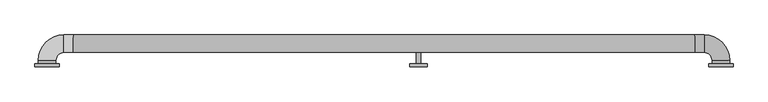
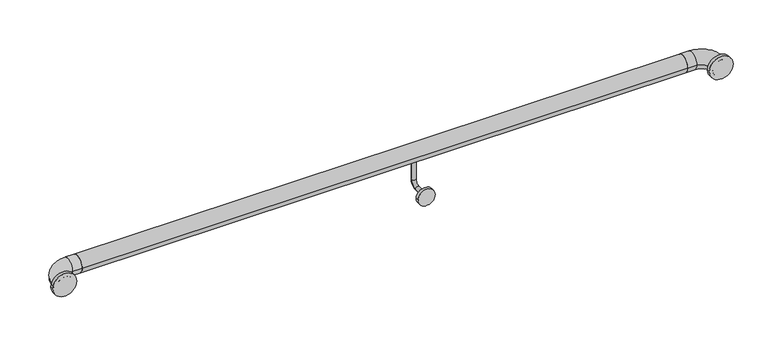
"""IFC4 building model written with IfcOpenShell, lengths in millimetres: railing geometry."""

from ifc_helpers import new_model, si_unit, point, frame, frame_2d, origin, place, context, project, spatial, circle_curve, ellipse_curve, trimmed, segment, composite_curve, outline, extrude, source, transform, mapped, element, save
from ifc_brep_helpers import plane_surface, cylinder_surface, revolved_surface, advanced_brep


def railing_d82230a8(model_context):
    return source(origin(), model_context, "Body", "SolidModel", [
        extrude(outline(composite_curve([segment(trimmed(circle_curve(frame_2d((32728.1400611, 874.6)), 25.4), [point((32753.5400611, 874.6))], [point((32702.7400611, 874.6))], False, "CARTESIAN"), True, "CONTINUOUS"), segment(trimmed(circle_curve(frame_2d((32728.1400611, 874.6)), 25.4), [point((32702.7400611, 874.6))], [point((32753.5400611, 874.6))], False, "CARTESIAN"), True, "CONTINUOUS")], self_intersect=False)), frame((9766.6129185, 0.0, 0.0), z_axis=(1.0, 0.0, 0.0), x_axis=(0.0, 1.0, 0.0)), (0.0, 0.0, 1.0), 1800.0),
        extrude(outline(composite_curve([segment(trimmed(circle_curve(frame_2d((773.2, 10766.6129185)), 25.4), [point((773.2, 10792.0129185))], [point((773.2, 10741.2129185))], False, "CARTESIAN"), True, "CONTINUOUS"), segment(trimmed(circle_curve(frame_2d((773.2, 10766.6129185)), 25.4), [point((773.2, 10741.2129185))], [point((773.2, 10792.0129185))], False, "CARTESIAN"), True, "CONTINUOUS")], self_intersect=False)), frame((0.0, 32661.1900611, 0.0), z_axis=(0.0, 1.0, 0.0), x_axis=(0.0, 0.0, 1.0)), (0.0, 0.0, 1.0), 9.525),
        advanced_brep(
        [(10760.2629185, 32728.1900611, 849.2), (10772.9629185, 32728.1900611, 849.2), (10760.2629185, 32728.1900611, 792.25), (10772.9629185, 32728.1900611, 792.25), (10772.9629185, 32709.1400611, 773.2), (10760.2629185, 32709.1400611, 773.2), (10760.2629185, 32670.7150611, 773.2), (10772.9629185, 32670.7150611, 773.2)],
        [
            (0, 1, circle_curve(frame((10766.6129185, 32728.1900611, 849.2), z_axis=(0.0, 0.0, 1.0), x_axis=(1.0, 0.0, 0.0)), 6.35)),
            (1, 0, circle_curve(frame((10766.6129185, 32728.1900611, 849.2), z_axis=(0.0, 0.0, 1.0), x_axis=(1.0, 0.0, 0.0)), 6.35)),
            (0, 2),
            (2, 3, circle_curve(frame((10766.6129185, 32728.1900611, 792.25), z_axis=(0.0, 0.0, 1.0), x_axis=(1.0, 0.0, 0.0)), 6.35)),
            (3, 1),
            (3, 2, circle_curve(frame((10766.6129185, 32728.1900611, 792.25), z_axis=(0.0, 0.0, 1.0), x_axis=(1.0, 0.0, 0.0)), 6.35)),
            (4, 3, circle_curve(frame((10772.9629185, 32709.1400611, 792.25), z_axis=(1.0, 0.0, 0.0), x_axis=(0.0, 1.0, 0.0)), 19.05)),
            (2, 5, circle_curve(frame((10760.2629185, 32709.1400611, 792.25), z_axis=(-1.0, 0.0, 0.0), x_axis=(0.0, 1.0, 0.0)), 19.05)),
            (5, 4, circle_curve(frame((10766.6129185, 32709.1400611, 773.2), z_axis=(0.0, 1.0, 0.0), x_axis=(1.0, 0.0, 0.0)), 6.35)),
            (4, 5, circle_curve(frame((10766.6129185, 32709.1400611, 773.2), z_axis=(0.0, 1.0, 0.0), x_axis=(1.0, 0.0, 0.0)), 6.35)),
            (6, 7, circle_curve(frame((10766.6129185, 32670.7150611, 773.2), z_axis=(0.0, -1.0, 0.0), x_axis=(1.0, 0.0, 0.0)), 6.35)),
            (7, 6, circle_curve(frame((10766.6129185, 32670.7150611, 773.2), z_axis=(0.0, -1.0, 0.0), x_axis=(1.0, 0.0, 0.0)), 6.35)),
            (5, 6),
            (7, 4),
        ],
        [
            plane_surface(frame((10772.9629185, 32728.1900611, 849.2), z_axis=(0.0, 0.0, 1.0), x_axis=(0.0, -1.0, 0.0))),
            cylinder_surface(frame((10766.6129185, 32728.1900611, 849.2), z_axis=(0.0, 0.0, 1.0), x_axis=(1.0, 0.0, 0.0)), 6.35),
            revolved_surface(trimmed(ellipse_curve(frame((10766.6129185, 32728.1900611, 792.25), z_axis=(0.0, 0.0, 1.0), x_axis=(1.0, 0.0, 0.0)), 6.35, 6.35), [point((10760.2629185, 32728.1900611, 792.25))], [point((10772.9629185, 32728.1900611, 792.25))], True, "CARTESIAN"), (10766.6129185, 32709.1400611, 792.25), (-1.0, 0.0, 0.0)),
            revolved_surface(trimmed(ellipse_curve(frame((10766.6129185, 32728.1900611, 792.25), z_axis=(0.0, 0.0, 1.0), x_axis=(1.0, 0.0, 0.0)), 6.35, 6.35), [point((10772.9629185, 32728.1900611, 792.25))], [point((10760.2629185, 32728.1900611, 792.25))], True, "CARTESIAN"), (10766.6129185, 32709.1400611, 792.25), (-1.0, 0.0, 0.0)),
            plane_surface(frame((10766.6129185, 32670.7150611, 766.85), z_axis=(0.0, -1.0, 0.0), x_axis=(1.0, 0.0, 0.0))),
            cylinder_surface(frame((10766.6129185, 32709.1400611, 773.2), z_axis=(0.0, 1.0, 0.0), x_axis=(1.0, 0.0, 0.0)), 6.35),
        ],
        [
            (0, [[1, 2]]),
            (1, [[-1, 3, 4, 5]]),
            (1, [[-2, -5, 6, -3]]),
            (2, [[7, -4, 8, 9]]),
            (3, [[-8, -6, -7, 10]]),
            (4, [[11, 12]]),
            (5, [[-9, 13, -12, 14]]),
            (5, [[-10, -14, -11, -13]]),
        ],
    ),
        extrude(outline(composite_curve([segment(trimmed(circle_curve(frame_2d((874.7, 11642.6129185)), 35.4), [point((874.7, 11678.0129185))], [point((874.7, 11607.2129185))], False, "CARTESIAN"), True, "CONTINUOUS"), segment(trimmed(circle_curve(frame_2d((874.7, 11642.6129185)), 35.4), [point((874.7, 11607.2129185))], [point((874.7, 11678.0129185))], False, "CARTESIAN"), True, "CONTINUOUS")], self_intersect=False)), frame((0.0, 32661.1900611, 0.0), z_axis=(0.0, 1.0, 0.0), x_axis=(0.0, 0.0, 1.0)), (0.0, 0.0, 1.0), 9.525),
        advanced_brep(
        [(11566.6129185, 32702.7900611, 874.7), (11566.6129185, 32753.5900611, 874.7), (11594.1129185, 32702.7900611, 874.7), (11594.1129185, 32753.5900611, 874.7), (11668.0129185, 32679.6900611, 874.7), (11617.2129185, 32679.6900611, 874.7), (11617.2129185, 32661.1900611, 874.7), (11668.0129185, 32661.1900611, 874.7)],
        [
            (0, 1, circle_curve(frame((11566.6129185, 32728.1900611, 874.7), z_axis=(-1.0, 0.0, 0.0), x_axis=(0.0, 1.0, 0.0)), 25.4)),
            (1, 0, circle_curve(frame((11566.6129185, 32728.1900611, 874.7), z_axis=(-1.0, 0.0, 0.0), x_axis=(0.0, 1.0, 0.0)), 25.4)),
            (0, 2),
            (2, 3, circle_curve(frame((11594.1129185, 32728.1900611, 874.7), z_axis=(-1.0, 0.0, 0.0), x_axis=(0.0, 1.0, 0.0)), 25.4)),
            (3, 1),
            (3, 2, circle_curve(frame((11594.1129185, 32728.1900611, 874.7), z_axis=(-1.0, 0.0, 0.0), x_axis=(0.0, 1.0, 0.0)), 25.4)),
            (4, 3, circle_curve(frame((11594.1129185, 32679.6900611, 874.7), z_axis=(0.0, 0.0, 1.0), x_axis=(0.0, 1.0, 0.0)), 73.9)),
            (2, 5, circle_curve(frame((11594.1129185, 32679.6900611, 874.7), z_axis=(0.0, 0.0, -1.0), x_axis=(0.0, 1.0, 0.0)), 23.1)),
            (5, 4, circle_curve(frame((11642.6129185, 32679.6900611, 874.7), z_axis=(0.0, 1.0, 0.0), x_axis=(1.0, 0.0, 0.0)), 25.4)),
            (4, 5, circle_curve(frame((11642.6129185, 32679.6900611, 874.7), z_axis=(0.0, 1.0, 0.0), x_axis=(1.0, 0.0, 0.0)), 25.4)),
            (6, 7, circle_curve(frame((11642.6129185, 32661.1900611, 874.7), z_axis=(0.0, -1.0, 0.0), x_axis=(1.0, 0.0, 0.0)), 25.4)),
            (7, 6, circle_curve(frame((11642.6129185, 32661.1900611, 874.7), z_axis=(0.0, -1.0, 0.0), x_axis=(1.0, 0.0, 0.0)), 25.4)),
            (5, 6),
            (7, 4),
        ],
        [
            plane_surface(frame((11566.6129185, 32728.1900611, 874.7), z_axis=(-1.0, 0.0, 0.0), x_axis=(0.0, 0.0, 1.0))),
            cylinder_surface(frame((11566.6129185, 32728.1900611, 874.7), z_axis=(-1.0, 0.0, 0.0), x_axis=(0.0, 1.0, 0.0)), 25.4),
            revolved_surface(trimmed(ellipse_curve(frame((11594.1129185, 32728.1900611, 874.7), z_axis=(-1.0, 0.0, 0.0), x_axis=(0.0, 1.0, 0.0)), 25.4, 25.4), [point((11594.1129185, 32702.7900611, 874.7))], [point((11594.1129185, 32753.5900611, 874.7))], True, "CARTESIAN"), (11594.1129185, 32679.6900611, 874.7), (0.0, 0.0, -1.0)),
            revolved_surface(trimmed(ellipse_curve(frame((11594.1129185, 32728.1900611, 874.7), z_axis=(-1.0, 0.0, 0.0), x_axis=(0.0, 1.0, 0.0)), 25.4, 25.4), [point((11594.1129185, 32753.5900611, 874.7))], [point((11594.1129185, 32702.7900611, 874.7))], True, "CARTESIAN"), (11594.1129185, 32679.6900611, 874.7), (0.0, 0.0, -1.0)),
            plane_surface(frame((11642.6129185, 32661.1900611, 874.7), z_axis=(0.0, -1.0, 0.0), x_axis=(0.0, 0.0, 1.0))),
            cylinder_surface(frame((11642.6129185, 32679.6900611, 874.7), z_axis=(0.0, 1.0, 0.0), x_axis=(1.0, 0.0, 0.0)), 25.4),
        ],
        [
            (0, [[1, 2]]),
            (1, [[-1, 3, 4, 5]]),
            (1, [[-2, -5, 6, -3]]),
            (2, [[7, -4, 8, 9]]),
            (3, [[-8, -6, -7, 10]]),
            (4, [[11, 12]]),
            (5, [[-9, 13, -12, 14]]),
            (5, [[-10, -14, -11, -13]]),
        ],
    ),
        extrude(outline(composite_curve([segment(trimmed(circle_curve(frame_2d((874.7, 9690.6129185)), 35.4), [point((874.7, 9726.0129185))], [point((874.7, 9655.2129185))], False, "CARTESIAN"), True, "CONTINUOUS"), segment(trimmed(circle_curve(frame_2d((874.7, 9690.6129185)), 35.4), [point((874.7, 9655.2129185))], [point((874.7, 9726.0129185))], False, "CARTESIAN"), True, "CONTINUOUS")], self_intersect=False)), frame((0.0, 32661.1900611, 0.0), z_axis=(0.0, 1.0, 0.0), x_axis=(0.0, 0.0, 1.0)), (0.0, 0.0, 1.0), 9.525),
        advanced_brep(
        [(9766.6129185, 32753.5900611, 874.7), (9766.6129185, 32702.7900611, 874.7), (9739.1129185, 32702.7900611, 874.7), (9739.1129185, 32753.5900611, 874.7), (9665.2129185, 32679.6900611, 874.7), (9716.0129185, 32679.6900611, 874.7), (9665.2129185, 32661.1900611, 874.7), (9716.0129185, 32661.1900611, 874.7)],
        [
            (0, 1, circle_curve(frame((9766.6129185, 32728.1900611, 874.7), z_axis=(1.0, 0.0, 0.0), x_axis=(0.0, -1.0, 0.0)), 25.4)),
            (1, 0, circle_curve(frame((9766.6129185, 32728.1900611, 874.7), z_axis=(1.0, 0.0, 0.0), x_axis=(0.0, -1.0, 0.0)), 25.4)),
            (1, 2),
            (2, 3, circle_curve(frame((9739.1129185, 32728.1900611, 874.7), z_axis=(1.0, 0.0, 0.0), x_axis=(0.0, -1.0, 0.0)), 25.4)),
            (3, 0),
            (3, 2, circle_curve(frame((9739.1129185, 32728.1900611, 874.7), z_axis=(1.0, 0.0, 0.0), x_axis=(0.0, -1.0, 0.0)), 25.4)),
            (4, 3, circle_curve(frame((9739.1129185, 32679.6900611, 874.7), z_axis=(0.0, 0.0, -1.0), x_axis=(0.0, 1.0, 0.0)), 73.9)),
            (2, 5, circle_curve(frame((9739.1129185, 32679.6900611, 874.7), z_axis=(0.0, 0.0, 1.0), x_axis=(0.0, 1.0, 0.0)), 23.1)),
            (5, 4, circle_curve(frame((9690.6129185, 32679.6900611, 874.7), z_axis=(0.0, 1.0, 0.0), x_axis=(1.0, 0.0, 0.0)), 25.4)),
            (4, 5, circle_curve(frame((9690.6129185, 32679.6900611, 874.7), z_axis=(0.0, 1.0, 0.0), x_axis=(1.0, 0.0, 0.0)), 25.4)),
            (6, 7, circle_curve(frame((9690.6129185, 32661.1900611, 874.7), z_axis=(0.0, -1.0, 0.0), x_axis=(1.0, 0.0, 0.0)), 25.4)),
            (7, 6, circle_curve(frame((9690.6129185, 32661.1900611, 874.7), z_axis=(0.0, -1.0, 0.0), x_axis=(1.0, 0.0, 0.0)), 25.4)),
            (5, 7),
            (6, 4),
        ],
        [
            plane_surface(frame((9766.6129185, 32728.1900611, 874.7), z_axis=(1.0, 0.0, 0.0), x_axis=(0.0, 0.0, 1.0))),
            cylinder_surface(frame((9766.6129185, 32728.1900611, 874.7), z_axis=(1.0, 0.0, 0.0), x_axis=(0.0, -1.0, 0.0)), 25.4),
            revolved_surface(trimmed(ellipse_curve(frame((9739.1129185, 32728.1900611, 874.7), z_axis=(1.0, 0.0, 0.0), x_axis=(0.0, -1.0, 0.0)), 25.4, 25.4), [point((9739.1129185, 32702.7900611, 874.7))], [point((9739.1129185, 32753.5900611, 874.7))], True, "CARTESIAN"), (9739.1129185, 32679.6900611, 874.7), (0.0, 0.0, 1.0)),
            revolved_surface(trimmed(ellipse_curve(frame((9739.1129185, 32728.1900611, 874.7), z_axis=(1.0, 0.0, 0.0), x_axis=(0.0, -1.0, 0.0)), 25.4, 25.4), [point((9739.1129185, 32753.5900611, 874.7))], [point((9739.1129185, 32702.7900611, 874.7))], True, "CARTESIAN"), (9739.1129185, 32679.6900611, 874.7), (0.0, 0.0, 1.0)),
            plane_surface(frame((9690.6129185, 32661.1900611, 874.7), z_axis=(0.0, -1.0, 0.0), x_axis=(0.0, 0.0, 1.0))),
            cylinder_surface(frame((9690.6129185, 32679.6900611, 874.7), z_axis=(0.0, 1.0, 0.0), x_axis=(1.0, 0.0, 0.0)), 25.4),
        ],
        [
            (0, [[1, 2]]),
            (1, [[-2, 3, 4, 5]]),
            (1, [[-1, -5, 6, -3]]),
            (2, [[7, -4, 8, 9]]),
            (3, [[-8, -6, -7, 10]]),
            (4, [[11, 12]]),
            (5, [[-9, 13, -11, 14]]),
            (5, [[-10, -14, -12, -13]]),
        ],
    ),
    ])


if __name__ == "__main__":
    model = new_model("IFC4")
    model_context = context("Model", 3, world=origin())
    ifc_project = project(units=[si_unit("LENGTHUNIT", "METRE", prefix="MILLI")], contexts=[model_context])
    site = spatial("IfcSite", under=ifc_project)
    building = spatial("IfcBuilding", under=site)
    placement = place(None, origin())
    railing_shape = railing_d82230a8(model_context)
    element("IfcRailing", 1, at=placement, inside=building, context=model_context, shape_type="MappedRepresentation", body=[
        mapped(railing_shape, transform((0.0, 0.0, 0.0), x_axis=(1.0, 0.0, 0.0), y_axis=(0.0, 1.0, 0.0), z_axis=(0.0, 0.0, 1.0))),
    ])
    save(model, "model.ifc")

# Revit data of these elements
# Element 1 (IfcRailing)
#   Materials on its faces: "Ferro - Pintura Esmalte"
# Materials
#   "Ferro - Pintura Esmalte": class "Pintura", colour RGB 255 255 255, transparency 0, Cost = 0
